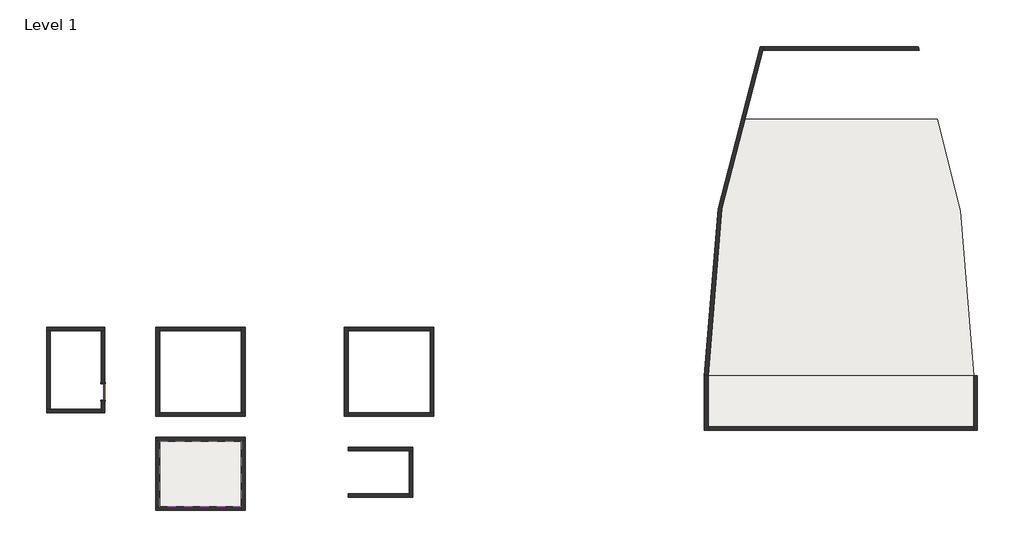
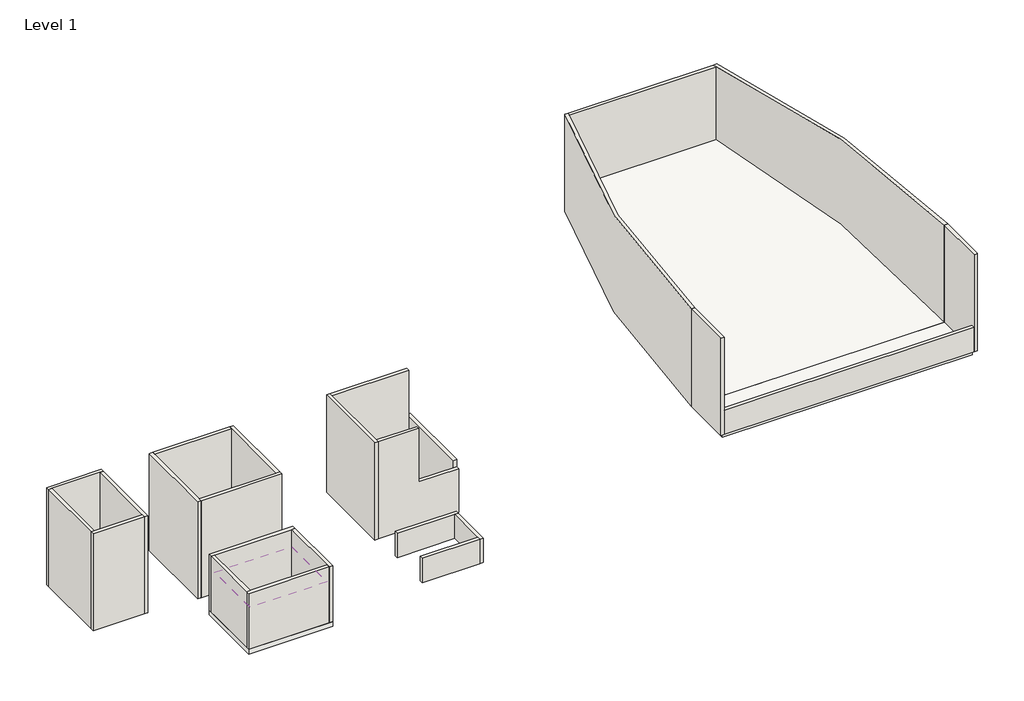
# One storey: 25 walls, 3 slabs, 1 covering, 1 door.
"""IFC4 building model written with IfcOpenShell, lengths in millimetres."""

import ifcopenshell
import ifcopenshell.guid

model = None  # the IFC model being written
_history = None  # IfcOwnerHistory: only IFC2X3 demands one
_inside = {}  # id of a spatial element -> (the spatial element, [elements in it])
_under = {}  # id of a project, library or spatial element -> (it, [spatial elements below it])
_declared = {}  # id of a project -> (the project, [libraries it declares])
_typed = {}  # id of a type object -> (the type object, [elements of that type])
_made_of = {}  # id of a material, layer set ... -> (it, [elements and type objects made of it])


def new_model(schema):
    """Start an empty IFC model of exactly this schema.

    Asked for "IFC4X3", IfcOpenShell would pick the latest addendum, in which some entities
    have other attributes; the version numbers below select the first issue.
    IFC2X3 requires an IfcOwnerHistory on every rooted entity: one is made here for all.
    """
    global model, _history
    if schema == "IFC4X3":
        model = ifcopenshell.file(schema_version=(4, 3, 0, 0))
    else:
        model = ifcopenshell.file(schema=schema)
    _inside.clear()
    _under.clear()
    _declared.clear()
    _typed.clear()
    _made_of.clear()
    _history = None
    if model.schema == "IFC2X3":
        org = make("IfcOrganization", Name="unknown")
        user = make(
            "IfcPersonAndOrganization",
            ThePerson=make("IfcPerson", FamilyName="unknown"),
            TheOrganization=org,
        )
        app = make(
            "IfcApplication",
            ApplicationDeveloper=org,
            Version="unknown",
            ApplicationFullName="unknown",
            ApplicationIdentifier="unknown",
        )
        _history = make(
            "IfcOwnerHistory",
            OwningUser=user,
            OwningApplication=app,
            ChangeAction="ADDED",
            CreationDate=0,
        )
    return model


def make(cls, **values):
    """One entity of the class cls with the attributes given. An attribute that is None is left unset."""
    return model.create_entity(
        cls, **{name: value for name, value in values.items() if value is not None}
    )


def rooted(cls, **values):
    """An entity with a GlobalId (a new one), such as an element, a storey or a relation."""
    return make(cls, GlobalId=ifcopenshell.guid.new(), OwnerHistory=_history, **values)


def si_unit(unit_type, name, prefix=None):
    """IfcSIUnit, for example si_unit("LENGTHUNIT", "METRE", prefix="MILLI")."""
    return make("IfcSIUnit", UnitType=unit_type, Prefix=prefix, Name=name)


def assignment(units):
    """IfcUnitAssignment: the units of a project."""
    return None if units is None else make("IfcUnitAssignment", Units=units)


def point(xyz):
    """IfcCartesianPoint."""
    return None if xyz is None else make("IfcCartesianPoint", Coordinates=xyz)


def direction(xyz):
    """IfcDirection."""
    return None if xyz is None else make("IfcDirection", DirectionRatios=xyz)


def frame(location, z_axis=None, x_axis=None):
    """IfcAxis2Placement3D, a coordinate frame: its origin and axes. An axis left out is left unset."""
    return make(
        "IfcAxis2Placement3D",
        Location=point(location),
        Axis=direction(z_axis),
        RefDirection=direction(x_axis),
    )


def frame_2d(location, x_axis=None):
    """IfcAxis2Placement2D, a coordinate frame in the plane: its origin and x axis."""
    return make(
        "IfcAxis2Placement2D", Location=point(location), RefDirection=direction(x_axis)
    )


def origin():
    """The frame at (0, 0, 0) with its axes left unset."""
    return frame((0.0, 0.0, 0.0))


def origin_with_axes():
    """The frame at (0, 0, 0) with the z axis (0, 0, 1) and the x axis (1, 0, 0) written out."""
    return frame((0.0, 0.0, 0.0), z_axis=(0.0, 0.0, 1.0), x_axis=(1.0, 0.0, 0.0))


def place(relative_to, where):
    """IfcLocalPlacement: puts the frame where relative to a parent placement (None: the world)."""
    return make(
        "IfcLocalPlacement", PlacementRelTo=relative_to, RelativePlacement=where
    )


def context(
    kind, dimensions, precision=None, world=None, true_north=None, identifier=None
):
    """IfcGeometricRepresentationContext, for example the 3D "Model" context."""
    return make(
        "IfcGeometricRepresentationContext",
        ContextIdentifier=identifier,
        ContextType=kind,
        CoordinateSpaceDimension=dimensions,
        Precision=precision,
        WorldCoordinateSystem=world,
        TrueNorth=true_north,
    )


def project(units=None, contexts=None):
    """IfcProject with its units and contexts."""
    return rooted(
        "IfcProject",
        Name="project",
        RepresentationContexts=contexts,
        UnitsInContext=assignment(units),
    )


def spatial(cls, under=None, at=None, **own):
    """A site, building, storey or space (cls), placed at a placement, below another one or the project."""
    s = rooted(cls, ObjectPlacement=at, **own)
    if under is not None:
        _under.setdefault(under.id(), (under, []))[1].append(s)
    return s


def polyline(points):
    """IfcPolyline through the points."""
    return make("IfcPolyline", Points=[point(p) for p in points])


def circle_curve(where, radius):
    """IfcCircle in the frame where."""
    return make("IfcCircle", Position=where, Radius=radius)


def ellipse_curve(where, semi_axis1, semi_axis2):
    """IfcEllipse in the frame where."""
    return make(
        "IfcEllipse", Position=where, SemiAxis1=semi_axis1, SemiAxis2=semi_axis2
    )


def trimmed(basis, trim1, trim2, sense, master):
    """IfcTrimmedCurve: the piece of a basis curve between two trims."""
    return make(
        "IfcTrimmedCurve",
        BasisCurve=basis,
        Trim1=trim1,
        Trim2=trim2,
        SenseAgreement=sense,
        MasterRepresentation=master,
    )


def segment(curve, same_sense, transition):
    """IfcCompositeCurveSegment."""
    return make(
        "IfcCompositeCurveSegment",
        Transition=transition,
        SameSense=same_sense,
        ParentCurve=curve,
    )


def composite_curve(segments, self_intersect=None):
    """IfcCompositeCurve: segments joined end to end."""
    return make("IfcCompositeCurve", Segments=segments, SelfIntersect=self_intersect)


def outline(outer, holes=None, kind="AREA"):
    """IfcArbitraryClosedProfileDef: a profile drawn as a closed curve; with holes, ...WithVoids."""
    if holes is None:
        return make("IfcArbitraryClosedProfileDef", ProfileType=kind, OuterCurve=outer)
    return make(
        "IfcArbitraryProfileDefWithVoids",
        ProfileType=kind,
        OuterCurve=outer,
        InnerCurves=holes,
    )


def extrude(swept, where, along, depth):
    """IfcExtrudedAreaSolid: the profile swept, set in the frame where, extruded along a direction by depth."""
    return make(
        "IfcExtrudedAreaSolid",
        SweptArea=swept,
        Position=where,
        ExtrudedDirection=direction(along),
        Depth=depth,
    )


def faces_of(points, faces, orient=None, outer=None):
    """IfcFace entities. A face is a list of loops; a loop is a list of indices into points, from 0.

    orient and outer hold one flag for each loop. By default every Orientation is true, the
    first loop of a face is its IfcFaceOuterBound and the others are IfcFaceBound.
    """
    made = []
    for i, loops in enumerate(faces):
        bounds = []
        for j, loop in enumerate(loops):
            is_outer = j == 0 if outer is None else outer[i][j]
            bounds.append(
                make(
                    "IfcFaceOuterBound" if is_outer else "IfcFaceBound",
                    Bound=make("IfcPolyLoop", Polygon=[points[k] for k in loop]),
                    Orientation=True if orient is None else orient[i][j],
                )
            )
        made.append(make("IfcFace", Bounds=bounds))
    return made


def faceted_brep(points, faces, orient=None, outer=None, voids=None):
    """IfcFacetedBrep: a solid bounded by flat faces; with voids (closed shells), ...WithVoids."""
    shared = [point(p) for p in points]
    hull = make("IfcClosedShell", CfsFaces=faces_of(shared, faces, orient, outer))
    if voids is None:
        return make("IfcFacetedBrep", Outer=hull)
    return make(
        "IfcFacetedBrepWithVoids",
        Outer=hull,
        Voids=[
            make(cls, CfsFaces=faces_of(shared, fs, o, b)) for cls, fs, o, b in voids
        ],
    )


def shape(context_of_items, identifier, shape_type, items):
    """IfcShapeRepresentation: the items that make up one representation, for example the "Body"."""
    return make(
        "IfcShapeRepresentation",
        ContextOfItems=context_of_items,
        RepresentationIdentifier=identifier,
        RepresentationType=shape_type,
        Items=items,
    )


def source(mapping_origin, context_of_items, identifier, shape_type, items):
    """IfcRepresentationMap: a shape defined once, which mapped items show again and again."""
    return make(
        "IfcRepresentationMap",
        MappingOrigin=mapping_origin,
        MappedRepresentation=shape(context_of_items, identifier, shape_type, items),
    )


def transform(
    local_origin,
    x_axis=None,
    y_axis=None,
    z_axis=None,
    scale=None,
    scale2=None,
    scale3=None,
    uniform=True,
):
    """IfcCartesianTransformationOperator3D, or its non-uniform kind. x_axis, y_axis, z_axis: its Axis1, 2, 3."""
    if uniform:
        return make(
            "IfcCartesianTransformationOperator3D",
            Axis1=direction(x_axis),
            Axis2=direction(y_axis),
            LocalOrigin=point(local_origin),
            Scale=scale,
            Axis3=direction(z_axis),
        )
    return make(
        "IfcCartesianTransformationOperator3DnonUniform",
        Axis1=direction(x_axis),
        Axis2=direction(y_axis),
        LocalOrigin=point(local_origin),
        Scale=scale,
        Axis3=direction(z_axis),
        Scale2=scale2,
        Scale3=scale3,
    )


def mapped(mapping_source, mapping_target):
    """IfcMappedItem: shows the shape of a source again, moved by a transform."""
    return make(
        "IfcMappedItem", MappingSource=mapping_source, MappingTarget=mapping_target
    )


def made_of(thing, what):
    """Note that an element or type object is made of a material, layer set ...; save() writes the relation."""
    if what is not None:
        _made_of.setdefault(what.id(), (what, []))[1].append(thing)
    return thing


def element(
    cls,
    number,
    at=None,
    inside=None,
    cuts=None,
    type_object=None,
    material=None,
    context=None,
    identifier="Body",
    shape_type=None,
    held_by="IfcProductDefinitionShape",
    body=None,
    shapes=None,
    **own,
):
    """One element of the class cls, such as IfcWall. Its Tag is "e" and its number.

    at: its placement. inside: the storey or other place that contains it. cuts: it is an
    opening in that element (IfcRelVoidsElement). A single representation is given by context,
    identifier, shape_type and body (its items); several are given by shapes. held_by: the class
    of the entity that holds the representations. save() writes the other relations.
    """
    e = rooted(cls, Tag="e%d" % number, ObjectPlacement=at, **own)
    if body is not None:
        shapes = [shape(context, identifier, shape_type, body)]
    if shapes is not None:
        e.Representation = make(held_by, Representations=shapes)
    if inside is not None:
        _inside.setdefault(inside.id(), (inside, []))[1].append(e)
    if cuts is not None:
        rooted(
            "IfcRelVoidsElement", RelatingBuildingElement=cuts, RelatedOpeningElement=e
        )
    if type_object is not None:
        _typed.setdefault(type_object.id(), (type_object, []))[1].append(e)
    return made_of(e, material)


def aggregate(whole, parts):
    """IfcRelAggregates: a whole, such as a stair, and the parts it consists of."""
    return rooted("IfcRelAggregates", RelatingObject=whole, RelatedObjects=parts)


def save(model, path):
    """Write the relations noted so far, then the file.

    IfcRelAggregates (storeys below a building ...), IfcRelContainedInSpatialStructure (elements
    in a storey), IfcRelDefinesByType, IfcRelAssociatesMaterial and IfcRelDeclares: one each for
    every whole, place, type object, material and project.
    """
    for whole, parts in _under.values():
        aggregate(whole, parts)
    for where, things in _inside.values():
        rooted(
            "IfcRelContainedInSpatialStructure",
            RelatedElements=things,
            RelatingStructure=where,
        )
    for kind, things in _typed.values():
        rooted("IfcRelDefinesByType", RelatedObjects=things, RelatingType=kind)
    for what, things in _made_of.values():
        rooted("IfcRelAssociatesMaterial", RelatedObjects=things, RelatingMaterial=what)
    for by, libraries in _declared.values():
        rooted("IfcRelDeclares", RelatingContext=by, RelatedDefinitions=libraries)
    model.write(path)


def plane_surface(at):
    """IfcPlane: the flat surface through the origin of the frame at, square to its z axis."""
    return make("IfcPlane", Position=at)


def cylinder_surface(at, radius):
    """IfcCylindricalSurface: all points at the distance radius from the z axis of the frame at."""
    return make("IfcCylindricalSurface", Position=at, Radius=radius)


def revolved_surface(curve, axis_point, axis_direction):
    """IfcSurfaceOfRevolution: the curve turned about the line through axis_point along axis_direction."""
    return make(
        "IfcSurfaceOfRevolution",
        SweptCurve=make("IfcArbitraryOpenProfileDef", ProfileType="CURVE", Curve=curve),
        AxisPosition=make("IfcAxis1Placement", Location=point(axis_point), Axis=direction(axis_direction)),
    )


def advanced_brep(points, edges, surfaces, faces):
    """IfcAdvancedBrep: a solid bounded by faces that lie on surfaces and meet in shared edges.

    An edge is (start, end): straight between two places in points (the first is 0);
    or (start, end, curve); or (start, end, curve, False) where it runs against its curve.
    A face is (place in surfaces, loops), or (place, loops, False) where it looks against
    its surface's normal. A loop lists edges by number (the first is 1), with a minus sign
    where the edge is run from its end to its start. The first loop is the outer one.
    """
    corners = [point(p) for p in points]
    vertices = [make("IfcVertexPoint", VertexGeometry=c) for c in corners]
    made = []
    for start, end, *more in edges:
        made.append(
            make(
                "IfcEdgeCurve",
                EdgeStart=vertices[start],
                EdgeEnd=vertices[end],
                EdgeGeometry=more[0] if more else make("IfcPolyline", Points=[corners[start], corners[end]]),
                SameSense=more[1] if len(more) > 1 else True,
            )
        )
    hull = []
    for where, loops, *sense in faces:
        bounds = []
        for j, loop in enumerate(loops):
            ring = [make("IfcOrientedEdge", EdgeElement=made[abs(k) - 1], Orientation=k > 0) for k in loop]
            bounds.append(
                make(
                    "IfcFaceOuterBound" if j == 0 else "IfcFaceBound",
                    Bound=make("IfcEdgeLoop", EdgeList=ring),
                    Orientation=True,
                )
            )
        hull.append(make("IfcAdvancedFace", Bounds=bounds, FaceSurface=surfaces[where], SameSense=sense[0] if sense else True))
    return make("IfcAdvancedBrep", Outer=make("IfcClosedShell", CfsFaces=hull))


def door_54dd4da4(model_context):
    return source(origin(), model_context, "Body", "SweptSolid", [
        extrude(outline(polyline([(2209.8, -533.4), (0.0, -533.4), (0.0, -457.2), (2133.6, -457.2), (2133.6, 457.2), (0.0, 457.2), (0.0, 533.4), (2209.8, 533.4), (2209.8, -533.4)])), frame((0.0, 101.6, 0.0), z_axis=(0.0, 1.0, 0.0), x_axis=(0.0, 0.0, 1.0)), (0.0, 0.0, 1.0), 25.4),
        extrude(outline(polyline([(2209.8, 533.4), (2209.8, -533.4), (0.0, -533.4), (0.0, -457.2), (2133.6, -457.2), (2133.6, 457.2), (0.0, 457.2), (0.0, 533.4), (2209.8, 533.4)])), frame((0.0, -127.0, 0.0), z_axis=(0.0, 1.0, 0.0), x_axis=(0.0, 0.0, 1.0)), (0.0, 0.0, 1.0), 25.4),
        extrude(outline(polyline([(457.2, 50.8), (-457.2, 50.8), (-457.2, 101.6), (457.2, 101.6), (457.2, 50.8)])), origin_with_axes(), (0.0, 0.0, 1.0), 2133.6),
    ])


model = new_model("IFC4")

# Units and contexts
model_context = context("Model", 3, world=origin())
ifc_project = project(units=[si_unit("LENGTHUNIT", "METRE", prefix="MILLI")], contexts=[model_context])

# Site, building, storey
site = spatial("IfcSite", under=ifc_project)
building = spatial("IfcBuilding", under=site)
storey = spatial("IfcBuildingStorey", under=building, Name="Level 1", Elevation=0.0)

# Covering
placement = place(None, origin())
element("IfcCovering", 1, ObjectType="2' x 4' ACT System", at=placement, inside=storey, context=model_context, shape_type="SweptSolid", body=[
    extrude(outline(polyline([(3202.0355998, -6643.9561607), (7774.0355998, -6643.9561607), (7774.0355998, -10301.5561607), (3202.0355998, -10301.5561607), (3202.0355998, -6643.9561607)])), frame((0.0, 0.0, 2438.4), z_axis=(0.0, 0.0, 1.0), x_axis=(1.0, 0.0, 0.0)), (0.0, 0.0, 1.0), 57.15),
])

# Door
door_shape = door_54dd4da4(model_context)
element("IfcDoor", 2, ObjectType="Single-Flush : 36\" x 84\"", at=placement, inside=storey, context=model_context, shape_type="MappedRepresentation", body=[
    mapped(door_shape, transform((52.4355998, -3900.7561607, 0.0), x_axis=(0.0, -1.0, 0.0), y_axis=(1.0, 0.0, 0.0), z_axis=(0.0, 0.0, 1.0))),
])

# Slabs
element("IfcSlab", 3, ObjectType="Generic - 12\"", at=placement, inside=storey, context=model_context, shape_type="SweptSolid", body=[
    extrude(outline(polyline([(7977.2355998, -6440.7561607), (7977.2355998, -10504.7561607), (2998.8355998, -10504.7561607), (2998.8355998, -6440.7561607), (7977.2355998, -6440.7561607)])), frame((0.0, 0.0, -304.8), z_axis=(0.0, 0.0, 1.0), x_axis=(1.0, 0.0, 0.0)), (0.0, 0.0, 1.0), 304.8),
])
element("IfcSlab", 4, ObjectType="Generic - 12\"", at=placement, inside=storey, context=model_context, shape_type="AdvancedBrep", body=[
    advanced_brep(
    [(36837.1507422, 15151.513064, 1218.1277364), (45573.3840243, 15151.513064, 1218.1277364), (48613.6434245, -2999.3760933, -305.7067974), (48613.6434245, -3001.3470145, -305.8722636), (45512.186933, -3001.3470145, -305.8722636), (36368.186933, -3001.3470145, -305.8722636), (33796.891342, -3001.3470145, -305.8722636), (33796.891342, -2999.3760933, -305.7067974), (36837.1507422, 15151.513064, 1524.0), (33796.891342, -2999.3760933, 0.1654661), (33796.891342, -3001.3470145, 0.0), (36368.186933, -3001.3470145, 0.0), (45512.186933, -3001.3470145, 0.0), (48613.6434245, -3001.3470145, 0.0), (48613.6434245, -2999.3760933, 0.1654661), (45573.3840243, 15151.513064, 1524.0)],
    [
        (0, 1),
        (1, 2, ellipse_curve(frame((-6046.8781275, -2824.9045996, -291.0592677), z_axis=(0.0, 0.08365940519908287, -0.9964944073710277), x_axis=(0.0, -0.9964944073710277, -0.08365940519908266)), 54853.0925971, 54660.8)),
        (2, 3),
        (3, 4),
        (4, 5),
        (5, 6),
        (6, 7),
        (7, 0, ellipse_curve(frame((88457.412894, -2824.9045996, -291.0592677), z_axis=(0.0, 0.08365940519908287, -0.9964944073710277), x_axis=(0.0, -0.9964944073710277, -0.08365940519908266)), 54853.0925971, 54660.8)),
        (8, 9, ellipse_curve(frame((88457.412894, -2824.9045996, 14.8129958), z_axis=(0.0, -0.08365940519908287, 0.9964944073710277), x_axis=(0.0, -0.9964944073710277, -0.08365940519908266)), 54853.0925971, 54660.8)),
        (9, 10),
        (10, 11),
        (11, 12),
        (12, 13),
        (13, 14),
        (14, 15, ellipse_curve(frame((-6046.8781275, -2824.9045996, 14.8129958), z_axis=(0.0, -0.08365940519908287, 0.9964944073710277), x_axis=(0.0, -0.9964944073710277, -0.08365940519908266)), 54853.0925971, 54660.8)),
        (15, 8),
        (0, 8),
        (15, 1),
        (14, 2),
        (13, 3),
        (12, 4),
        (11, 5),
        (10, 6),
        (9, 7),
    ],
    [
        plane_surface(frame((41205.2673832, 15151.513064, 1218.1277364), z_axis=(0.0, 0.08365940519908287, -0.9964944073710277), x_axis=(0.0, -0.9964944073710277, -0.08365940519908287))),
        plane_surface(frame((41205.2673832, 15151.513064, 1524.0), z_axis=(0.0, -0.08365940519908287, 0.9964944073710277), x_axis=(0.0, 0.9964944073710277, 0.08365940519908287))),
        plane_surface(frame((36837.1507422, 15151.513064, 1218.1277364), z_axis=(0.0, 1.0, 0.0), x_axis=(0.0, 0.0, 1.0))),
        cylinder_surface(frame((-6046.8781275, -2824.9045996, 0.0), z_axis=(0.0, 0.0, -1.0), x_axis=(1.0, 0.0, 0.0)), 54660.8),
        plane_surface(frame((48613.6434245, -2999.3760933, -305.7067974), z_axis=(1.0, 0.0, 0.0), x_axis=(0.0, 0.0, 1.0))),
        plane_surface(frame((48613.6434245, -3001.3470145, -305.8722636), z_axis=(0.0, -1.0, 0.0), x_axis=(0.0, 0.0, 1.0))),
        plane_surface(frame((45512.186933, -3001.3470145, -305.8722636), z_axis=(0.0, -1.0, 0.0), x_axis=(0.0, 0.0, 1.0))),
        plane_surface(frame((36368.186933, -3001.3470145, -305.8722636), z_axis=(0.0, -1.0, 0.0), x_axis=(0.0, 0.0, 1.0))),
        plane_surface(frame((33796.891342, -3001.3470145, -305.8722636), z_axis=(-1.0, 0.0, 0.0), x_axis=(0.0, 0.0, 1.0))),
        cylinder_surface(frame((88457.412894, -2824.9045996, 0.0), z_axis=(0.0, 0.0, -1.0), x_axis=(1.0, 0.0, 0.0)), 54660.8),
    ],
    [
        (0, [[1, 2, 3, 4, 5, 6, 7, 8]]),
        (1, [[9, 10, 11, 12, 13, 14, 15, 16]]),
        (2, [[-1, 17, -16, 18]]),
        (3, [[-2, -18, -15, 19]]),
        (4, [[-3, -19, -14, 20]]),
        (5, [[-4, -20, -13, 21]]),
        (6, [[-5, -21, -12, 22]]),
        (7, [[-6, -22, -11, 23]]),
        (8, [[-7, -23, -10, 24]]),
        (9, [[-8, -24, -9, -17]]),
    ],
),
])
element("IfcSlab", 5, ObjectType="Generic - 12\"", at=placement, inside=storey, context=model_context, shape_type="SweptSolid", body=[
    extrude(outline(polyline([(48613.6434245, -3001.3470145), (48613.6434245, -5846.1470145), (33796.891342, -5846.1470145), (33796.891342, -3001.3470145), (48613.6434245, -3001.3470145)])), frame((0.0, 0.0, -304.8), z_axis=(0.0, 0.0, 1.0), x_axis=(1.0, 0.0, 0.0)), (0.0, 0.0, 1.0), 304.8),
])

# Walls
element("IfcWall", 6, ObjectType="Generic - 8\"", at=placement, inside=storey, context=model_context, shape_type="Brep", body=[
    faceted_brep([(-3097.1644002, -497.1561607, 0.0), (-2893.9644002, -497.1561607, 0.0), (-49.1644002, -497.1561607, 0.0), (154.0355998, -497.1561607, 0.0), (154.0355998, -497.1561607, 6096.0), (-49.1644002, -497.1561607, 6096.0), (-2893.9644002, -497.1561607, 6096.0), (-3097.1644002, -497.1561607, 6096.0), (-3097.1644002, -293.9561607, 0.0), (-3097.1644002, -293.9561607, 6096.0), (154.0355998, -293.9561607, 6096.0), (154.0355998, -293.9561607, 0.0)], [[[0, 1, 2, 3, 4, 5, 6, 7]], [[8, 9, 10, 11]], [[3, 2, 1, 0, 8, 11]], [[7, 6, 5, 4, 10, 9]], [[4, 3, 11, 10]], [[0, 7, 9, 8]]]),
])
element("IfcWall", 7, ObjectType="Generic - 8\"", at=placement, inside=storey, context=model_context, shape_type="Brep", body=[
    faceted_brep([(-49.1644002, -4357.9561607, 2133.6), (-49.1644002, -4357.9561607, 0.0), (-49.1644002, -4865.9561607, 0.0), (-49.1644002, -5069.1561607, 0.0), (-49.1644002, -5069.1561607, 6096.0), (-49.1644002, -4865.9561607, 6096.0), (-49.1644002, -497.1561607, 6096.0), (-49.1644002, -497.1561607, 0.0), (-49.1644002, -3443.5561607, 0.0), (-49.1644002, -3443.5561607, 2133.6), (154.0355998, -5069.1561607, 0.0), (154.0355998, -4357.9561607, 0.0), (154.0355998, -4357.9561607, 2133.6), (154.0355998, -3443.5561607, 2133.6), (154.0355998, -3443.5561607, 0.0), (154.0355998, -497.1561607, 0.0), (154.0355998, -497.1561607, 6096.0), (154.0355998, -5069.1561607, 6096.0)], [[[0, 1, 2, 3, 4, 5, 6, 7, 8, 9]], [[10, 11, 12, 13, 14, 15, 16, 17]], [[8, 7, 15, 14]], [[3, 2, 1, 11, 10]], [[6, 5, 4, 17, 16]], [[7, 6, 16, 15]], [[4, 3, 10, 17]], [[12, 11, 1, 0]], [[13, 12, 0, 9]], [[14, 13, 9, 8]]]),
])
element("IfcWall", 8, ObjectType="Generic - 8\"", at=placement, inside=storey, context=model_context, shape_type="Brep", body=[
    faceted_brep([(-49.1644002, -4865.9561607, 0.0), (-2893.9644002, -4865.9561607, 0.0), (-3097.1644002, -4865.9561607, 0.0), (-3097.1644002, -4865.9561607, 6096.0), (-2893.9644002, -4865.9561607, 6096.0), (-49.1644002, -4865.9561607, 6096.0), (-49.1644002, -5069.1561607, 0.0), (-49.1644002, -5069.1561607, 6096.0), (-3097.1644002, -5069.1561607, 6096.0), (-3097.1644002, -5069.1561607, 0.0)], [[[0, 1, 2, 3, 4, 5]], [[6, 7, 8, 9]], [[2, 1, 0, 6, 9]], [[5, 4, 3, 8, 7]], [[0, 5, 7, 6]], [[3, 2, 9, 8]]]),
])
element("IfcWall", 9, ObjectType="Generic - 8\"", at=placement, inside=storey, context=model_context, shape_type="SweptSolid", body=[
    extrude(outline(polyline([(-2893.9644002, -497.1561607), (-2893.9644002, -4865.9561607), (-3097.1644002, -4865.9561607), (-3097.1644002, -497.1561607), (-2893.9644002, -497.1561607)])), origin_with_axes(), (0.0, 0.0, 1.0), 6096.0),
])
element("IfcWall", 10, ObjectType="Generic - 8\"", at=placement, inside=storey, context=model_context, shape_type="Brep", body=[
    faceted_brep([(2998.8355998, -293.9561607, 0.0), (2998.8355998, -5272.3561607, 0.0), (2998.8355998, -5272.3561607, 6096.0), (2998.8355998, -293.9561607, 6096.0), (3202.0355998, -293.9561607, 0.0), (3202.0355998, -293.9561607, 6096.0), (3202.0355998, -497.1561607, 6096.0), (3202.0355998, -5069.1561607, 6096.0), (3202.0355998, -5272.3561607, 6096.0), (3202.0355998, -5272.3561607, 0.0), (3202.0355998, -5069.1561607, 0.0), (3202.0355998, -497.1561607, 0.0)], [[[0, 1, 2, 3]], [[4, 5, 6, 7, 8, 9, 10, 11]], [[1, 0, 4, 11, 10, 9]], [[3, 2, 8, 7, 6, 5]], [[2, 1, 9, 8]], [[0, 3, 5, 4]]]),
])
element("IfcWall", 11, ObjectType="Generic - 8\"", at=placement, inside=storey, context=model_context, shape_type="Brep", body=[
    faceted_brep([(3202.0355998, -5272.3561607, 0.0), (7977.2355998, -5272.3561607, 0.0), (7977.2355998, -5272.3561607, 6096.0), (3202.0355998, -5272.3561607, 6096.0), (3202.0355998, -5069.1561607, 0.0), (3202.0355998, -5069.1561607, 6096.0), (7774.0355998, -5069.1561607, 6096.0), (7977.2355998, -5069.1561607, 6096.0), (7977.2355998, -5069.1561607, 0.0), (7774.0355998, -5069.1561607, 0.0)], [[[0, 1, 2, 3]], [[4, 5, 6, 7, 8, 9]], [[1, 0, 4, 9, 8]], [[3, 2, 7, 6, 5]], [[0, 3, 5, 4]], [[2, 1, 8, 7]]]),
])
element("IfcWall", 12, ObjectType="Generic - 8\"", at=placement, inside=storey, context=model_context, shape_type="Brep", body=[
    faceted_brep([(7977.2355998, -5069.1561607, 0.0), (7977.2355998, -293.9561607, 0.0), (7977.2355998, -293.9561607, 6096.0), (7977.2355998, -5069.1561607, 6096.0), (7774.0355998, -5069.1561607, 0.0), (7774.0355998, -5069.1561607, 6096.0), (7774.0355998, -497.1561607, 6096.0), (7774.0355998, -293.9561607, 6096.0), (7774.0355998, -293.9561607, 0.0), (7774.0355998, -497.1561607, 0.0)], [[[0, 1, 2, 3]], [[4, 5, 6, 7, 8, 9]], [[1, 0, 4, 9, 8]], [[3, 2, 7, 6, 5]], [[0, 3, 5, 4]], [[2, 1, 8, 7]]]),
])
element("IfcWall", 13, ObjectType="Generic - 8\"", at=placement, inside=storey, context=model_context, shape_type="SweptSolid", body=[
    extrude(outline(polyline([(3202.0355998, -293.9561607), (7774.0355998, -293.9561607), (7774.0355998, -497.1561607), (3202.0355998, -497.1561607), (3202.0355998, -293.9561607)])), origin_with_axes(), (0.0, 0.0, 1.0), 6096.0),
])
element("IfcWall", 14, ObjectType="Generic - 8\"", at=placement, inside=storey, context=model_context, shape_type="Brep", body=[
    faceted_brep([(2998.8355998, -6643.9561607, 0.0), (3202.0355998, -6643.9561607, 0.0), (7774.0355998, -6643.9561607, 0.0), (7977.2355998, -6643.9561607, 0.0), (7977.2355998, -6643.9561607, 3505.2), (7774.0355998, -6643.9561607, 3505.2), (3202.0355998, -6643.9561607, 3505.2), (2998.8355998, -6643.9561607, 3505.2), (2998.8355998, -6440.7561607, 0.0), (2998.8355998, -6440.7561607, 3505.2), (7977.2355998, -6440.7561607, 3505.2), (7977.2355998, -6440.7561607, 0.0)], [[[0, 1, 2, 3, 4, 5, 6, 7]], [[8, 9, 10, 11]], [[3, 2, 1, 0, 8, 11]], [[7, 6, 5, 4, 10, 9]], [[4, 3, 11, 10]], [[0, 7, 9, 8]]]),
])
element("IfcWall", 15, ObjectType="Generic - 8\"", at=placement, inside=storey, context=model_context, shape_type="Brep", body=[
    faceted_brep([(7774.0355998, -6643.9561607, 0.0), (7774.0355998, -10301.5561607, 0.0), (7774.0355998, -10504.7561607, 0.0), (7774.0355998, -10504.7561607, 3505.2), (7774.0355998, -10301.5561607, 3505.2), (7774.0355998, -6643.9561607, 3505.2), (7977.2355998, -6643.9561607, 0.0), (7977.2355998, -6643.9561607, 3505.2), (7977.2355998, -10504.7561607, 3505.2), (7977.2355998, -10504.7561607, 0.0)], [[[0, 1, 2, 3, 4, 5]], [[6, 7, 8, 9]], [[2, 1, 0, 6, 9]], [[5, 4, 3, 8, 7]], [[0, 5, 7, 6]], [[3, 2, 9, 8]]]),
])
element("IfcWall", 16, ObjectType="Generic - 8\"", at=placement, inside=storey, context=model_context, shape_type="Brep", body=[
    faceted_brep([(7774.0355998, -10301.5561607, 0.0), (3202.0355998, -10301.5561607, 0.0), (2998.8355998, -10301.5561607, 0.0), (2998.8355998, -10301.5561607, 3505.2), (3202.0355998, -10301.5561607, 3505.2), (7774.0355998, -10301.5561607, 3505.2), (7774.0355998, -10504.7561607, 0.0), (7774.0355998, -10504.7561607, 3505.2), (2998.8355998, -10504.7561607, 3505.2), (2998.8355998, -10504.7561607, 0.0)], [[[0, 1, 2, 3, 4, 5]], [[6, 7, 8, 9]], [[2, 1, 0, 6, 9]], [[5, 4, 3, 8, 7]], [[0, 5, 7, 6]], [[3, 2, 9, 8]]]),
])
element("IfcWall", 17, ObjectType="Generic - 8\"", at=placement, inside=storey, context=model_context, shape_type="SweptSolid", body=[
    extrude(outline(polyline([(3202.0355998, -6643.9561607), (3202.0355998, -10301.5561607), (2998.8355998, -10301.5561607), (2998.8355998, -6643.9561607), (3202.0355998, -6643.9561607)])), origin_with_axes(), (0.0, 0.0, 1.0), 3505.2),
])
element("IfcWall", 18, ObjectType="Generic - 8\"", at=placement, inside=storey, context=model_context, shape_type="Brep", body=[
    faceted_brep([(13514.4355998, -293.9561607, 0.0), (13514.4355998, -5272.3561607, 0.0), (13514.4355998, -5272.3561607, 6096.0), (13514.4355998, -293.9561607, 6096.0), (13717.6355998, -293.9561607, 0.0), (13717.6355998, -293.9561607, 6096.0), (13717.6355998, -497.1561607, 6096.0), (13717.6355998, -5069.1561607, 6096.0), (13717.6355998, -5272.3561607, 6096.0), (13717.6355998, -5272.3561607, 0.0), (13717.6355998, -5069.1561607, 0.0), (13717.6355998, -497.1561607, 0.0)], [[[0, 1, 2, 3]], [[4, 5, 6, 7, 8, 9, 10, 11]], [[1, 0, 4, 11, 10, 9]], [[3, 2, 8, 7, 6, 5]], [[2, 1, 9, 8]], [[0, 3, 5, 4]]]),
])
element("IfcWall", 19, ObjectType="Generic - 8\"", at=placement, inside=storey, context=model_context, shape_type="Brep", body=[
    faceted_brep([(13717.6355998, -5272.3561607, 0.0), (18492.8355998, -5272.3561607, 0.0), (18492.8355998, -5272.3561607, 2743.2), (16105.2355998, -5272.3561607, 2743.2), (16105.2355998, -5272.3561607, 6096.0), (13717.6355998, -5272.3561607, 6096.0), (13717.6355998, -5069.1561607, 0.0), (13717.6355998, -5069.1561607, 6096.0), (16105.2355998, -5069.1561607, 6096.0), (16105.2355998, -5069.1561607, 2743.2), (18492.8355998, -5069.1561607, 2743.2), (18492.8355998, -5069.1561607, 0.0), (18289.6355998, -5069.1561607, 0.0)], [[[0, 1, 2, 3, 4, 5]], [[6, 7, 8, 9, 10, 11, 12]], [[0, 5, 7, 6]], [[2, 1, 11, 10]], [[1, 0, 6, 12, 11]], [[5, 4, 8, 7]], [[3, 2, 10, 9]], [[4, 3, 9, 8]]]),
])
element("IfcWall", 20, ObjectType="Generic - 8\"", at=placement, inside=storey, context=model_context, shape_type="Brep", body=[
    faceted_brep([(18492.8355998, -5069.1561607, 0.0), (18492.8355998, -293.9561607, 0.0), (18492.8355998, -293.9561607, 3200.4), (18492.8355998, -5069.1561607, 3200.4), (18492.8355998, -5069.1561607, 2743.2), (18289.6355998, -5069.1561607, 0.0), (18289.6355998, -5069.1561607, 3200.4), (18289.6355998, -293.9561607, 3200.4), (18289.6355998, -293.9561607, 0.0), (18289.6355998, -497.1561607, 0.0)], [[[0, 1, 2, 3, 4]], [[5, 6, 7, 8, 9]], [[1, 0, 5, 9, 8]], [[0, 4, 3, 6, 5]], [[2, 1, 8, 7]], [[3, 2, 7, 6]]]),
])
element("IfcWall", 21, ObjectType="Generic - 8\"", at=placement, inside=storey, context=model_context, shape_type="Brep", body=[
    faceted_brep([(18289.6355998, -293.9561607, 0.0), (13717.6355998, -293.9561607, 0.0), (13717.6355998, -293.9561607, 6096.0), (18289.6355998, -293.9561607, 6096.0), (18289.6355998, -293.9561607, 3200.4), (18289.6355998, -497.1561607, 0.0), (18289.6355998, -497.1561607, 6096.0), (13717.6355998, -497.1561607, 6096.0), (13717.6355998, -497.1561607, 0.0)], [[[0, 1, 2, 3, 4]], [[5, 6, 7, 8]], [[1, 0, 5, 8]], [[3, 2, 7, 6]], [[2, 1, 8, 7]], [[0, 4, 3, 6, 5]]]),
])
element("IfcWall", 22, ObjectType="Generic - 8\"", at=placement, inside=storey, context=model_context, shape_type="AdvancedBrep", body=[
    advanced_brep(
    [(48816.8434245, -2999.7000898, 6096.0), (45717.5884264, 15354.713064, 6096.0), (45502.1718952, 15354.713064, 6096.0), (45573.3872797, 15151.5034631, 6096.0), (48613.6434245, -2999.3760933, 6096.0), (48816.8434245, -2999.7000898, 0.0), (48613.6434245, -2999.3760933, 0.0), (45573.3872797, 15151.5034631, 0.0), (45502.1718952, 15354.713064, 0.0), (45717.5884264, 15354.713064, 0.0)],
    [
        (0, 1, circle_curve(frame((-6046.8781275, -2824.9045996, 6096.0), z_axis=(0.0, 0.0, 1.0), x_axis=(1.0, 0.0, 0.0)), 54864.0)),
        (1, 2),
        (2, 3, circle_curve(frame((-6046.8781275, -2824.9045996, 6096.0), z_axis=(0.0, 0.0, -1.0), x_axis=(1.0, 0.0, 0.0)), 54660.8)),
        (3, 4, circle_curve(frame((-6046.8781275, -2824.9045996, 6096.0), z_axis=(0.0, 0.0, -1.0), x_axis=(1.0, 0.0, 0.0)), 54660.7999168)),
        (4, 0),
        (5, 6),
        (6, 7, circle_curve(frame((-6046.8781275, -2824.9045996, 0.0), z_axis=(0.0, 0.0, 1.0), x_axis=(1.0, 0.0, 0.0)), 54660.8)),
        (7, 8, circle_curve(frame((-6046.8781275, -2824.9045996, 0.0), z_axis=(0.0, 0.0, 1.0), x_axis=(1.0, 0.0, 0.0)), 54660.7999168)),
        (8, 9),
        (9, 5, circle_curve(frame((-6046.8781275, -2824.9045996, 0.0), z_axis=(0.0, 0.0, -1.0), x_axis=(1.0, 0.0, 0.0)), 54864.0)),
        (0, 5),
        (9, 1),
        (2, 8),
        (6, 4),
    ],
    [
        plane_surface(frame((48817.1218725, -2824.9045996, 6096.0), z_axis=(0.0, 0.0, 1.0), x_axis=(0.0, 1.0, 0.0))),
        plane_surface(frame((48817.1218725, -2824.9045996, 0.0), z_axis=(0.0, 0.0, -1.0), x_axis=(0.0, -1.0, 0.0))),
        cylinder_surface(frame((-6046.8781275, -2824.9045996, 0.0), z_axis=(0.0, 0.0, 1.0), x_axis=(1.0, 0.0, 0.0)), 54864.0),
        revolved_surface(polyline([(48613.9218725, -2824.9045996, 0.0), (48613.9218725, -2824.9045996, 6096.0)]), (-6046.8781275, -2824.9045996, 0.0), (0.0, 0.0, -1.0)),
        plane_surface(frame((48613.6434245, -2999.3760933, 0.0), z_axis=(-0.0015944686883487965, -0.9999987288339931, 0.0), x_axis=(0.9999987288339931, -0.0015944686883487965, 0.0))),
        plane_surface(frame((36764.9982559, 15354.713064, 0.0), z_axis=(0.0, 1.0, 0.0), x_axis=(-1.0, 0.0, 0.0))),
    ],
    [
        (0, [[1, 2, 3, 4, 5]]),
        (1, [[6, 7, 8, 9, 10]]),
        (2, [[-1, 11, -10, 12]]),
        (3, [[-4, -3, 13, -8, -7, 14]]),
        (4, [[-5, -14, -6, -11]]),
        (5, [[-2, -12, -9, -13]]),
    ],
),
])
element("IfcWall", 23, ObjectType="Generic - 8\"", at=placement, inside=storey, context=model_context, shape_type="Brep", body=[
    faceted_brep([(48613.6434245, -2999.3760933, 0.0), (48613.6434245, -5846.1470145, 0.0), (48613.6434245, -6049.3470145, 0.0), (48613.6434245, -6049.3470145, 1524.0), (48613.6434245, -6049.3470145, 6096.0), (48613.6434245, -5846.1470145, 6096.0), (48613.6434245, -2999.3760933, 6096.0), (48816.8434245, -2999.7000898, 0.0), (48816.8434245, -2999.7000898, 6096.0), (48816.8434245, -6049.3470145, 6096.0), (48816.8434245, -6049.3470145, 0.0), (48802.4946674, -6049.3470145, 6096.0)], [[[0, 1, 2, 3, 4, 5, 6]], [[7, 8, 9, 10]], [[2, 1, 0, 7, 10]], [[6, 5, 4, 11, 9, 8]], [[0, 6, 8, 7]], [[2, 10, 9, 11, 4, 3]]]),
])
element("IfcWall", 24, ObjectType="Generic - 8\"", at=placement, inside=storey, context=model_context, shape_type="AdvancedBrep", body=[
    advanced_brep(
    [(33796.891342, -2999.3760933, 6096.0), (36837.1474868, 15151.5034631, 6096.0), (36908.3628713, 15354.713064, 6096.0), (36692.9463401, 15354.713064, 6096.0), (33593.691342, -2999.7000898, 6096.0), (33796.891342, -2999.3760933, 0.0), (33593.691342, -2999.7000898, 0.0), (36692.9463401, 15354.713064, 0.0), (36908.3628713, 15354.713064, 0.0), (36837.1474868, 15151.5034631, 0.0)],
    [
        (0, 1, circle_curve(frame((88457.412894, -2824.9045996, 6096.0), z_axis=(0.0, 0.0, -1.0), x_axis=(-1.0, 0.0, 0.0)), 54660.8)),
        (1, 2, circle_curve(frame((88457.412894, -2824.9045996, 6096.0), z_axis=(0.0, 0.0, -1.0), x_axis=(-1.0, 0.0, 0.0)), 54660.7999168)),
        (2, 3),
        (3, 4, circle_curve(frame((88457.412894, -2824.9045996, 6096.0), z_axis=(0.0, 0.0, 1.0), x_axis=(-1.0, 0.0, 0.0)), 54864.0)),
        (4, 0),
        (5, 6),
        (6, 7, circle_curve(frame((88457.412894, -2824.9045996, 0.0), z_axis=(0.0, 0.0, -1.0), x_axis=(-1.0, 0.0, 0.0)), 54864.0)),
        (7, 8),
        (8, 9, circle_curve(frame((88457.412894, -2824.9045996, 0.0), z_axis=(0.0, 0.0, 1.0), x_axis=(-1.0, 0.0, 0.0)), 54660.8)),
        (9, 5, circle_curve(frame((88457.412894, -2824.9045996, 0.0), z_axis=(0.0, 0.0, 1.0), x_axis=(-1.0, 0.0, 0.0)), 54660.7999168)),
        (0, 5),
        (8, 2),
        (3, 7),
        (6, 4),
    ],
    [
        plane_surface(frame((33796.612894, -2824.9045996, 6096.0), z_axis=(0.0, 0.0, 1.0), x_axis=(0.0, 1.0, 0.0))),
        plane_surface(frame((33796.612894, -2824.9045996, 0.0), z_axis=(0.0, 0.0, -1.0), x_axis=(0.0, -1.0, 0.0))),
        revolved_surface(polyline([(33796.61289399999, -2824.9045996, 0.0), (33796.61289399999, -2824.9045996, 6096.0)]), (88457.412894, -2824.9045996, 0.0), (0.0, 0.0, -1.0)),
        cylinder_surface(frame((88457.412894, -2824.9045996, 0.0), z_axis=(0.0, 0.0, 1.0), x_axis=(-1.0, 0.0, 0.0)), 54864.0),
        plane_surface(frame((33593.691342, -2999.7000898, 0.0), z_axis=(0.001594468715108758, -0.9999987288339504, 0.0), x_axis=(0.9999987288339504, 0.001594468715108758, 0.0))),
        plane_surface(frame((36764.9982559, 15354.713064, 0.0), z_axis=(0.0, 1.0, 0.0), x_axis=(-1.0, 0.0, 0.0))),
    ],
    [
        (0, [[1, 2, 3, 4, 5]]),
        (1, [[6, 7, 8, 9, 10]]),
        (2, [[-2, -1, 11, -10, -9, 12]]),
        (3, [[-4, 13, -7, 14]]),
        (4, [[-5, -14, -6, -11]]),
        (5, [[-3, -12, -8, -13]]),
    ],
),
])
element("IfcWall", 25, ObjectType="Generic - 8\"", at=placement, inside=storey, context=model_context, shape_type="Brep", body=[
    faceted_brep([(33593.691342, -2999.7000898, 0.0), (33593.691342, -6049.3470145, 0.0), (33593.691342, -6049.3470145, 6096.0), (33593.691342, -2999.7000898, 6096.0), (33796.891342, -2999.3760933, 0.0), (33796.891342, -2999.3760933, 6096.0), (33796.891342, -5846.1470145, 6096.0), (33796.891342, -6049.3470145, 6096.0), (33796.891342, -6049.3470145, 1524.0), (33796.891342, -6049.3470145, 0.0), (33796.891342, -5846.1470145, 0.0), (33608.0401885, -6049.3470145, 6096.0)], [[[0, 1, 2, 3]], [[4, 5, 6, 7, 8, 9, 10]], [[1, 0, 4, 10, 9]], [[3, 2, 11, 7, 6, 5]], [[0, 3, 5, 4]], [[1, 9, 8, 7, 11, 2]]]),
])
element("IfcWall", 26, ObjectType="Generic - 8\"", at=placement, inside=storey, context=model_context, shape_type="SweptSolid", body=[
    extrude(outline(composite_curve([segment(polyline([(45573.3840243, 15151.513064), (36837.1507422, 15151.513064)]), True, "CONTINUOUS"), segment(trimmed(circle_curve(frame_2d((88457.412894, -2824.9045996)), 54660.8), [point((36837.1507422, 15151.513064))], [point((36908.3628713, 15354.713064))], False, "CARTESIAN"), True, "CONTINUOUS"), segment(polyline([(36908.3628713, 15354.713064), (45502.1718952, 15354.713064)]), True, "CONTINUOUS"), segment(trimmed(circle_curve(frame_2d((-6046.8781275, -2824.9045996)), 54660.8), [point((45502.1718952, 15354.713064))], [point((45573.3840243, 15151.513064))], False, "CARTESIAN"), True, "CONTINUOUS")], self_intersect=False)), origin_with_axes(), (0.0, 0.0, 1.0), 6096.0),
])
element("IfcWall", 27, ObjectType="Generic - 8\"", at=placement, inside=storey, context=model_context, shape_type="Brep", body=[
    faceted_brep([(33796.891342, -6049.3470145, 0.0), (48613.6434245, -6049.3470145, 0.0), (48613.6434245, -6049.3470145, 1524.0), (45777.2673832, -6049.3470145, 1524.0), (36633.2673832, -6049.3470145, 1524.0), (33796.891342, -6049.3470145, 1524.0), (33796.891342, -5846.1470145, 0.0), (33796.891342, -5846.1470145, 1524.0), (36633.2673832, -5846.1470145, 1524.0), (45777.2673832, -5846.1470145, 1524.0), (48613.6434245, -5846.1470145, 1524.0), (48613.6434245, -5846.1470145, 0.0)], [[[0, 1, 2, 3, 4, 5]], [[6, 7, 8, 9, 10, 11]], [[1, 0, 6, 11]], [[5, 4, 3, 2, 10, 9, 8, 7]], [[0, 5, 7, 6]], [[2, 1, 11, 10]]]),
])
element("IfcWall", 28, ObjectType="Generic - 8\"", at=placement, inside=storey, context=model_context, shape_type="Brep", body=[
    faceted_brep([(13717.6355998, -7190.0486659, 0.0), (17134.7988188, -7190.0486659, 0.0), (17337.9988188, -7190.0486659, 0.0), (17337.9988188, -7190.0486659, 1524.0), (17134.7988188, -7190.0486659, 1524.0), (13717.6355998, -7190.0486659, 1524.0), (13717.6355998, -6986.8486659, 0.0), (13717.6355998, -6986.8486659, 1524.0), (17337.9988188, -6986.8486659, 1524.0), (17337.9988188, -6986.8486659, 0.0)], [[[0, 1, 2, 3, 4, 5]], [[6, 7, 8, 9]], [[2, 1, 0, 6, 9]], [[5, 4, 3, 8, 7]], [[0, 5, 7, 6]], [[3, 2, 9, 8]]]),
])
element("IfcWall", 29, ObjectType="Generic - 8\"", at=placement, inside=storey, context=model_context, shape_type="Brep", body=[
    faceted_brep([(17134.7988188, -7190.0486659, 0.0), (17134.7988188, -9577.6486659, 0.0), (17134.7988188, -9780.8486659, 0.0), (17134.7988188, -9780.8486659, 1524.0), (17134.7988188, -9577.6486659, 1524.0), (17134.7988188, -7190.0486659, 1524.0), (17337.9988188, -7190.0486659, 0.0), (17337.9988188, -7190.0486659, 1524.0), (17337.9988188, -9780.8486659, 1524.0), (17337.9988188, -9780.8486659, 0.0)], [[[0, 1, 2, 3, 4, 5]], [[6, 7, 8, 9]], [[2, 1, 0, 6, 9]], [[5, 4, 3, 8, 7]], [[0, 5, 7, 6]], [[3, 2, 9, 8]]]),
])
element("IfcWall", 30, ObjectType="Generic - 8\"", at=placement, inside=storey, context=model_context, shape_type="SweptSolid", body=[
    extrude(outline(polyline([(13717.6355998, -9577.6486659), (17134.7988188, -9577.6486659), (17134.7988188, -9780.8486659), (13717.6355998, -9780.8486659), (13717.6355998, -9577.6486659)])), origin_with_axes(), (0.0, 0.0, 1.0), 1524.0),
])

save(model, "model.ifc")

# Revit data of these elements
# Project information
#   Project Issue Date = "Issue Date"
#   Project Status = "Project Status"
#   Client Name = "Owner"
#   Project Address = "Enter address here"
#   Project Name = "Project Name"
#   Project Number = "Project Number"
# Type "2' x 4' ACT System"
#   Assembly Code = "C3030210"
#   built-in parameter 1002203 = 1 (stored number, unit not read)
#   built-in parameter 1002202 = 1 (stored number, unit not read)
#   Layers, outside or top first: 0' - 1 5/8" "Default" (function 1); 0' - 0 5/8" "Acoustic Ceiling Tile 24 x 48" (function 5)
# Type "Single-Flush : 36\" x 84\""
#   Type Mark = "1"
#   Construction Type Id = "MDOOR"
#   Assembly Code = "C1020"
#   Analytic Construction = "Metal"
#   Thickness = 0' - 2"
#   Heat Transfer Coefficient (U) = 3.7021 W/(m²·K)
#   Height = 7' - 0"
#   Trim Projection Ext = 0' - 1"
#   Trim Projection Int = 0' - 1"
#   Trim Width = 0' - 3"
#   Width = 3' - 0"
#   Door Material = Door - Panel
#   Frame Material = Door - Frame
#   Visual Light Transmittance = 0
#   Solar Heat Gain Coefficient = 0
#   Function = (empty or 0)
#   Wall Closure = (empty or 0)
# Type "Generic - 12\""
#   Assembly Code = "B1010"
#   Function = 0
#   Layers, outside or top first: 1' - 0" no material (function 1)
# Type "Generic - 8\""
#   Assembly Code = "B2010"
#   Layers, outside or top first: 0' - 8" no material (function 1)
# Element 1 (IfcCovering, "2' x 4' ACT System")
#   Height Offset From Level = 8' - 0"
#   Phase Created = New Construction
#   Materials on its faces: "Acoustic Ceiling Tile 24 x 48", "Default"
# Element 2 (IfcDoor, "Single-Flush : 36\" x 84\"")
#   Phase Created = New Construction
#   Materials on its faces: "Door - Frame", "Door - Panel"
# Elements 3, 4, 5 (IfcSlab, "Generic - 12\"")
#   Height Offset From Level = 0' - 0"
#   Phase Created = New Construction
#   Materials on its faces: "Default Floor"
# Elements 6, 7, 8, 9 (IfcWall, "Generic - 8\"")
#   Top Offset = 0' - 0"
#   Base Offset = 0' - 0"
#   wall height = 20' - 0"
#   Phase Created = New Construction
#   Base Constraint = Level 1
#   Top Constraint = Level 3
#   Materials on its faces: "Default Wall"
# Elements 10, 11, 12, 13, 19, 21 (IfcWall, "Generic - 8\"")
#   Top Offset = 0' - 0"
#   Base Offset = 0' - 0"
#   Unconnected Height = 20' - 0"
#   wall height = 20' - 0"
#   Phase Created = New Construction
#   Base Constraint = Level 1
#   Materials on its faces: "Default Wall"
# Elements 14, 15, 16, 17 (IfcWall, "Generic - 8\"")
#   Top Offset = 0' - 0"
#   Base Offset = 0' - 0"
#   wall height = 11' - 6"
#   Phase Created = New Construction
#   Base Constraint = Level 1
#   Top Constraint = Level 2
#   Materials on its faces: "Default Wall"
# Elements 18, 23, 25, 26 (IfcWall, "Generic - 8\"")
#   Top Offset = 0' - 0"
#   Base Offset = 0' - 0"
#   Unconnected Height = 20' - 0"
#   wall height = 20' - 0"
#   Phase Created = New Construction
#   Base Constraint = Level 1
#   Top Constraint = Level 3
#   Materials on its faces: "Default Wall"
# Element 20 (IfcWall, "Generic - 8\"")
#   Top Offset = 0' - 0"
#   Base Offset = 0' - 0"
#   wall height = 10' - 6"
#   Phase Created = New Construction
#   Base Constraint = Level 1
#   Top Constraint = Level 2
#   Materials on its faces: "Default Wall"
# Elements 22, 24 (IfcWall, "Generic - 8\"")
#   Top Offset = 0' - 0"
#   Base Offset = 0' - 0"
#   Unconnected Height = 20' - 0"
#   wall height = 20' - 0"
#   Phase Created = New Construction
#   Materials on its faces: "Default Wall"
# Elements 27, 28, 29, 30 (IfcWall, "Generic - 8\"")
#   Top Offset = 0' - 0"
#   Base Offset = 0' - 0"
#   wall height = 5' - 0"
#   Phase Created = New Construction
#   Base Constraint = Level 1
#   Top Constraint = Stage
#   Materials on its faces: "Default Wall"
# Materials
#   "Default": class "Miscellaneous", colour RGB 127 127 127, transparency 0, Cost = 0
#   "Acoustic Ceiling Tile 24 x 48": class "Generic", colour RGB 229 229 229, transparency 0, Description = "Acoustic Ceiling Tile 24 x 48", Cost = 0
#   "Door - Panel": class "Wood", colour RGB 210 159 95, transparency 0, Cost = 0
#   "Door - Frame": class "Miscellaneous", colour RGB 118 70 51, transparency 0, Cost = 0
#   "Default Floor": class "Miscellaneous", colour RGB 128 128 128, transparency 0, Cost = 0
#   "Default Wall": class "Miscellaneous", colour RGB 128 128 128, transparency 0, Cost = 0
# Room at (41143.02, 5941.216) mm, phase "New Construction", upper level "Level 3", upper offset 10' - 0", lower offset 0' - 0"
#   Number = "10017"
#   Name = "Seating"
# Room, not placed, phase "New Construction", upper offset 0' - 0", lower offset 0' - 0"
#   Number = "10019"
#   Name = "Room"
# Room at (-1549.751, -2556.717) mm, phase "New Construction", upper level "Level 1", upper offset 10' - 0", lower offset 0' - 0"
#   Number = "1"
#   Name = "My Room"
# Room at (5429.891, -1399.125) mm, phase "New Construction", upper level "Level 1", upper offset 10' - 0", lower offset 0' - 0"
#   Number = "10014"
#   Name = "Custom Name Room"
# Room at (5430.163, -8557.358) mm, phase "New Construction", upper level "Level 1", upper offset 10' - 0", lower offset 0' - 0"
#   Number = "10015"
#   Name = "Room with ceiling"
# Room at (15945.491, -1399.125) mm, phase "New Construction", upper level "Level 3", upper offset 10' - 0", lower offset 0' - 0"
#   Number = "10016"
#   Name = "Custom Name Room"
